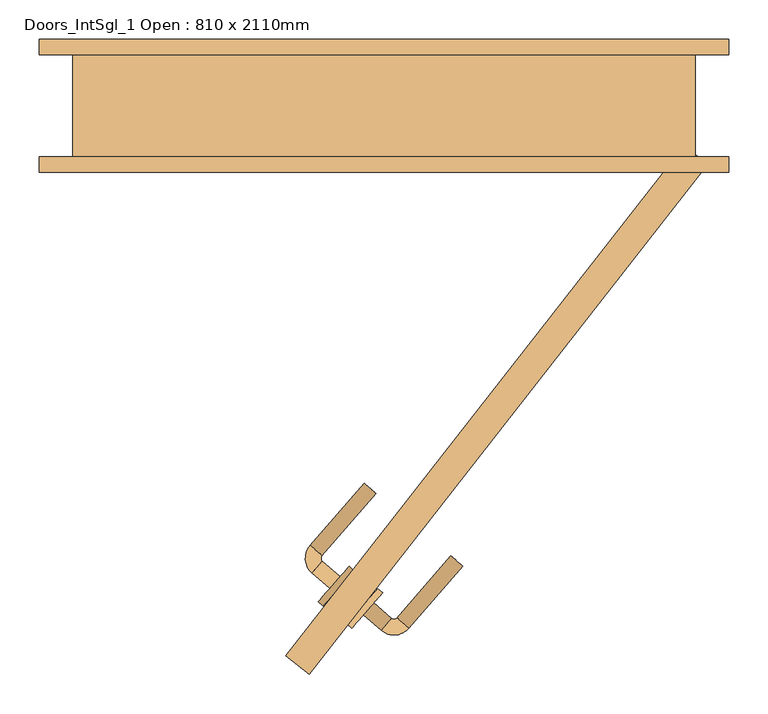
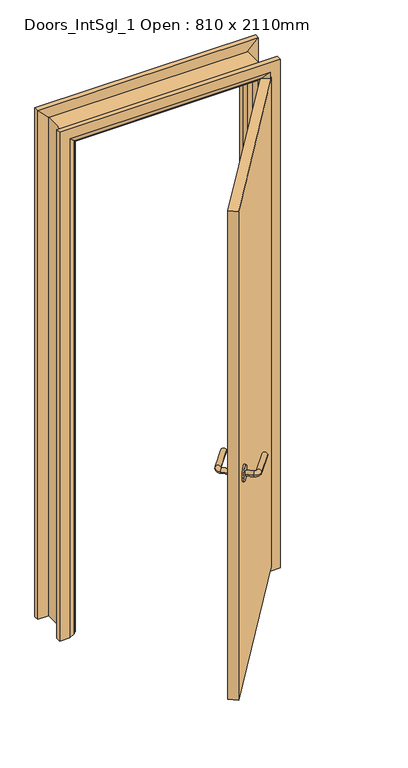
"""IFC4 building model written with IfcOpenShell, lengths in millimetres: door geometry, Doors_IntSgl_1 Open : 810 x 2110mm."""

from ifc_helpers import new_model, si_unit, point, frame, frame_2d, origin, place, context, project, spatial, polyline, circle_curve, ellipse_curve, trimmed, segment, composite_curve, outline, extrude, faceted_brep, source, transform, mapped, element, save
from ifc_brep_helpers import plane_surface, cylinder_surface, revolved_surface, advanced_brep


def doors_intsgl_1_open_810_x_2110mm_3496c895(model_context):
    return source(origin(), model_context, "Body", "SolidModel", [
        advanced_brep(
        [(-69.1197704, -615.7042456, 900.0), (-55.9985898, -600.610054, 900.0), (-91.7610578, -596.0224748, 900.0), (-78.6398772, -580.9282832, 900.0), (-79.13313, -573.8744401, 900.0), (-94.2273216, -560.7532595, 900.0), (-25.3411235, -481.5087536, 900.0), (-10.2469319, -494.6299342, 900.0)],
        [
            (0, 1, circle_curve(frame((-62.5591801, -608.1571498, 900.0), z_axis=(0.7547095802227883, -0.6560590289904886, 0.0), x_axis=(0.6560590289904885, 0.7547095802227881, 0.0)), 10.0)),
            (1, 0, circle_curve(frame((-62.5591801, -608.1571498, 900.0), z_axis=(0.7547095802227883, -0.6560590289904886, 0.0), x_axis=(0.6560590289904885, 0.7547095802227881, 0.0)), 10.0)),
            (0, 2),
            (2, 3, circle_curve(frame((-85.2004675, -588.475379, 900.0), z_axis=(0.7547095802227883, -0.6560590289904886, 0.0), x_axis=(0.6560590289904885, 0.7547095802227881, 0.0)), 10.0)),
            (3, 1),
            (3, 2, circle_curve(frame((-85.2004675, -588.475379, 900.0), z_axis=(0.7547095802227883, -0.6560590289904886, 0.0), x_axis=(0.6560590289904885, 0.7547095802227881, 0.0)), 10.0)),
            (4, 3, circle_curve(frame((-75.3595821, -577.1547353, 900.0), z_axis=(0.0, 0.0, 1.0), x_axis=(-0.6560590289904885, -0.7547095802227881, 0.0)), 5.0)),
            (2, 5, circle_curve(frame((-75.3595821, -577.1547353, 900.0), z_axis=(0.0, 0.0, -1.0), x_axis=(-0.6560590289904885, -0.7547095802227881, 0.0)), 25.0)),
            (5, 4, circle_curve(frame((-86.6802258, -567.3138498, 900.0), z_axis=(-0.656059028990488, -0.7547095802227886, 0.0), x_axis=(0.7547095802227886, -0.656059028990488, 0.0)), 10.0)),
            (4, 5, circle_curve(frame((-86.6802258, -567.3138498, 900.0), z_axis=(-0.6560590289904857, -0.7547095802227904, 0.0), x_axis=(0.7547095802227904, -0.6560590289904857, 0.0)), 10.0)),
            (6, 7, circle_curve(frame((-17.7940277, -488.0693439, 900.0), z_axis=(0.6560590289904886, 0.7547095802227883, 0.0), x_axis=(0.7547095802227881, -0.6560590289904885, 0.0)), 10.0)),
            (7, 6, circle_curve(frame((-17.7940277, -488.0693439, 900.0), z_axis=(0.6560590289904886, 0.7547095802227883, 0.0), x_axis=(0.7547095802227881, -0.6560590289904885, 0.0)), 10.0)),
            (5, 6),
            (7, 4),
        ],
        [
            plane_surface(frame((-62.5591801, -608.1571498, 900.0), z_axis=(0.7547095802227883, -0.6560590289904886, 0.0), x_axis=(0.0, 0.0, 1.0))),
            cylinder_surface(frame((-62.5591801, -608.1571498, 900.0), z_axis=(0.7547095802227881, -0.6560590289904885, 0.0), x_axis=(0.6560590289904885, 0.7547095802227881, 0.0)), 10.0),
            revolved_surface(trimmed(ellipse_curve(frame((-85.2004675, -588.475379, 900.0), z_axis=(0.7547095802227881, -0.6560590289904885, 0.0), x_axis=(0.6560590289904885, 0.7547095802227881, 0.0)), 10.0, 10.0), [point((-91.7610578, -596.0224748, 900.0))], [point((-78.6398772, -580.9282832, 900.0))], True, "CARTESIAN"), (-75.3595821, -577.1547353, 900.0), (0.0, 0.0, -1.0)),
            revolved_surface(trimmed(ellipse_curve(frame((-85.2004675, -588.475379, 900.0), z_axis=(0.7547095802227881, -0.6560590289904885, 0.0), x_axis=(0.6560590289904885, 0.7547095802227881, 0.0)), 10.0, 10.0), [point((-78.6398772, -580.9282832, 900.0))], [point((-91.7610578, -596.0224748, 900.0))], True, "CARTESIAN"), (-75.3595821, -577.1547353, 900.0), (0.0, 0.0, -1.0)),
            plane_surface(frame((-17.7940277, -488.0693439, 900.0), z_axis=(0.6560590289904886, 0.7547095802227883, 0.0), x_axis=(0.0, 0.0, 1.0))),
            cylinder_surface(frame((-86.6802258, -567.3138498, 900.0), z_axis=(-0.6560590289904885, -0.7547095802227881, 0.0), x_axis=(0.7547095802227881, -0.6560590289904885, 0.0)), 10.0),
        ],
        [
            (0, [[1, 2]]),
            (1, [[-1, 3, 4, 5]]),
            (1, [[-2, -5, 6, -3]]),
            (2, [[7, -4, 8, 9]]),
            (3, [[-8, -6, -7, 10]]),
            (4, [[11, 12]]),
            (5, [[-9, 13, -12, 14]]),
            (5, [[-10, -14, -11, -13]]),
        ],
    ),
        extrude(outline(composite_curve([segment(trimmed(circle_curve(frame_2d((0.0, -30.0)), 30.0), [point((0.0, -60.0))], [point((0.0, 0.0))], False, "CARTESIAN"), True, "CONTINUOUS"), segment(trimmed(circle_curve(frame_2d((0.0, -30.0)), 30.0), [point((0.0, 0.0))], [point((0.0, -60.0))], False, "CARTESIAN"), True, "CONTINUOUS")], self_intersect=False)), frame((-38.4798801, -592.6511086, 900.0), z_axis=(-0.7547095802227883, 0.6560590289904886, 0.0), x_axis=(0.0, 0.0, 1.0)), (0.0, 0.0, 1.0), 8.0),
        advanced_brep(
        [(-26.2647476, -649.3053178, 900.0), (-13.143567, -634.2111262, 900.0), (9.4977204, -653.8928971, 900.0), (-3.6234602, -668.9870887, 900.0), (16.5515634, -653.3996443, 900.0), (31.645755, -666.5208249, 900.0), (100.5319531, -587.276319, 900.0), (85.4377615, -574.1551384, 900.0)],
        [
            (0, 1, circle_curve(frame((-19.7041573, -641.758222, 900.0), z_axis=(-0.7547095802227883, 0.6560590289904886, 0.0), x_axis=(0.6560590289904885, 0.7547095802227881, 0.0)), 10.0)),
            (1, 0, circle_curve(frame((-19.7041573, -641.758222, 900.0), z_axis=(-0.7547095802227883, 0.6560590289904886, 0.0), x_axis=(0.6560590289904885, 0.7547095802227881, 0.0)), 10.0)),
            (1, 2),
            (2, 3, circle_curve(frame((2.9371301, -661.4399929, 900.0), z_axis=(-0.7547095802227883, 0.6560590289904886, 0.0), x_axis=(0.6560590289904885, 0.7547095802227881, 0.0)), 10.0)),
            (3, 0),
            (3, 2, circle_curve(frame((2.9371301, -661.4399929, 900.0), z_axis=(-0.7547095802227883, 0.6560590289904886, 0.0), x_axis=(0.6560590289904885, 0.7547095802227881, 0.0)), 10.0)),
            (4, 5, circle_curve(frame((24.0986592, -659.9602346, 900.0), z_axis=(-0.6560590289904913, -0.7547095802227858, 0.0), x_axis=(-0.7547095802227858, 0.6560590289904913, 0.0)), 10.0)),
            (5, 3, circle_curve(frame((12.7780155, -650.1193492, 900.0), z_axis=(0.0, 0.0, -1.0), x_axis=(-0.6560590289904885, -0.7547095802227881, 0.0)), 25.0)),
            (2, 4, circle_curve(frame((12.7780155, -650.1193492, 900.0), z_axis=(0.0, 0.0, 1.0), x_axis=(-0.6560590289904885, -0.7547095802227881, 0.0)), 5.0)),
            (5, 4, circle_curve(frame((24.0986592, -659.9602346, 900.0), z_axis=(-0.6560590289904891, -0.7547095802227877, 0.0), x_axis=(-0.7547095802227877, 0.6560590289904891, 0.0)), 10.0)),
            (6, 7, circle_curve(frame((92.9848573, -580.7157287, 900.0), z_axis=(0.6560590289904886, 0.7547095802227883, 0.0), x_axis=(-0.7547095802227881, 0.6560590289904885, 0.0)), 10.0)),
            (7, 6, circle_curve(frame((92.9848573, -580.7157287, 900.0), z_axis=(0.6560590289904886, 0.7547095802227883, 0.0), x_axis=(-0.7547095802227881, 0.6560590289904885, 0.0)), 10.0)),
            (4, 7),
            (6, 5),
        ],
        [
            plane_surface(frame((-19.7041573, -641.758222, 900.0), z_axis=(-0.7547095802227883, 0.6560590289904886, 0.0), x_axis=(0.0, 0.0, 1.0))),
            cylinder_surface(frame((-19.7041573, -641.758222, 900.0), z_axis=(-0.7547095802227881, 0.6560590289904885, 0.0), x_axis=(0.6560590289904885, 0.7547095802227881, 0.0)), 10.0),
            revolved_surface(trimmed(ellipse_curve(frame((2.9371301, -661.4399929, 900.0), z_axis=(0.7547095802227881, -0.6560590289904885, 0.0), x_axis=(0.6560590289904885, 0.7547095802227881, 0.0)), 10.0, 10.0), [point((-3.6234602, -668.9870887, 900.0))], [point((9.4977204, -653.8928971, 900.0))], True, "CARTESIAN"), (12.7780155, -650.1193492, 900.0), (0.0, 0.0, -1.0)),
            revolved_surface(trimmed(ellipse_curve(frame((2.9371301, -661.4399929, 900.0), z_axis=(0.7547095802227881, -0.6560590289904885, 0.0), x_axis=(0.6560590289904885, 0.7547095802227881, 0.0)), 10.0, 10.0), [point((9.4977204, -653.8928971, 900.0))], [point((-3.6234602, -668.9870887, 900.0))], True, "CARTESIAN"), (12.7780155, -650.1193492, 900.0), (0.0, 0.0, -1.0)),
            plane_surface(frame((92.9848573, -580.7157287, 900.0), z_axis=(0.6560590289904886, 0.7547095802227883, 0.0), x_axis=(0.0, 0.0, 1.0))),
            cylinder_surface(frame((24.0986592, -659.9602346, 900.0), z_axis=(-0.6560590289904885, -0.7547095802227881, 0.0), x_axis=(-0.7547095802227881, 0.6560590289904885, 0.0)), 10.0),
        ],
        [
            (0, [[1, 2]]),
            (1, [[3, 4, 5, -2]]),
            (1, [[-5, 6, -3, -1]]),
            (2, [[7, 8, -4, 9]]),
            (3, [[10, -9, -6, -8]]),
            (4, [[11, 12]]),
            (5, [[13, -11, 14, -7]]),
            (5, [[-14, -12, -13, -10]]),
        ],
    ),
        extrude(outline(composite_curve([segment(trimmed(circle_curve(frame_2d((0.0, 30.0)), 30.0), [point((0.0, 60.0))], [point((0.0, 0.0))], False, "CARTESIAN"), True, "CONTINUOUS"), segment(trimmed(circle_curve(frame_2d((0.0, 30.0)), 30.0), [point((0.0, 0.0))], [point((0.0, 60.0))], False, "CARTESIAN"), True, "CONTINUOUS")], self_intersect=False)), frame((-1.662534, -621.0037086, 900.0), z_axis=(-0.7547095802227883, 0.6560590289904886, 0.0), x_axis=(0.0, 0.0, -1.0)), (0.0, 0.0, 1.0), 8.0),
        extrude(outline(polyline([(383.3995748, -51.0018026), (413.3439834, -74.3969387), (-95.1923952, -725.2938212), (-125.1368039, -701.8986851), (383.3995748, -51.0018026)])), frame((0.0, 0.0, 18.0), z_axis=(0.0, 0.0, 1.0), x_axis=(1.0, 0.0, 0.0)), (0.0, 0.0, 1.0), 2060.0),
        advanced_brep(
        [(440.0, -85.0, 0.0), (400.0, -85.0, 0.0), (374.0, -71.0, 0.0), (370.0, -65.0, 0.0), (440.0, -65.0, 0.0), (440.0, -65.0, 2145.0), (440.0, -85.0, 2145.0), (370.0, -65.0, 2075.0), (-370.0, -65.0, 2075.0), (-370.0, -65.0, 0.0), (-440.0, -65.0, 0.0), (-440.0, -65.0, 2145.0), (374.0, -71.0, 2079.0), (400.0, -85.0, 2105.0), (-440.0, -85.0, 2145.0), (-440.0, -85.0, 0.0), (-400.0, -85.0, 0.0), (-400.0, -85.0, 2105.0), (-374.0, -71.0, 0.0), (-374.0, -71.0, 2079.0)],
        [
            (0, 1),
            (1, 2),
            (2, 3, circle_curve(frame((378.0, -64.0, 0.0), z_axis=(0.0, 0.0, -1.0), x_axis=(1.0, 0.0, 0.0)), 8.0622577)),
            (3, 4),
            (4, 0),
            (4, 5),
            (5, 6),
            (6, 0),
            (3, 7),
            (7, 8),
            (8, 9),
            (9, 10),
            (10, 11),
            (11, 5),
            (2, 12),
            (12, 7, ellipse_curve(frame((378.0, -64.0, 2083.0), z_axis=(0.7071067811865475, 0.0, -0.7071067811865475), x_axis=(-0.7071067811865474, 0.0, -0.7071067811865476)), 11.4017543, 8.0622577)),
            (1, 13),
            (13, 12),
            (6, 14),
            (14, 15),
            (15, 16),
            (16, 17),
            (17, 13),
            (10, 15),
            (14, 11),
            (9, 18, circle_curve(frame((-378.0, -64.0, 0.0), z_axis=(0.0, 0.0, -1.0), x_axis=(-1.0, 0.0, 0.0)), 8.0622577)),
            (18, 16),
            (19, 18),
            (8, 19, ellipse_curve(frame((-378.0, -64.0, 2083.0), z_axis=(-0.7071067811865475, 0.0, -0.7071067811865475), x_axis=(-0.7071067811865474, 0.0, 0.7071067811865476)), 11.4017543, 8.0622577)),
            (19, 17),
            (12, 19),
        ],
        [
            plane_surface(frame((370.0, -65.0, 0.0), z_axis=(0.0, 0.0, -1.0), x_axis=(0.0, 1.0, 0.0))),
            plane_surface(frame((440.0, -85.0, 0.0), z_axis=(1.0, 0.0, 0.0), x_axis=(0.0, 0.0, 1.0))),
            plane_surface(frame((440.0, -65.0, 0.0), z_axis=(0.0, 1.0, 0.0), x_axis=(0.0, 0.0, 1.0))),
            cylinder_surface(frame((378.0, -64.0, 0.0), z_axis=(0.0, 0.0, -1.0), x_axis=(1.0, 0.0, 0.0)), 8.0622577),
            plane_surface(frame((374.0, -71.0, 0.0), z_axis=(-0.4740998230350126, -0.880471099922178, 0.0), x_axis=(0.0, 0.0, 1.0))),
            plane_surface(frame((400.0, -85.0, 0.0), z_axis=(0.0, -1.0, 0.0), x_axis=(0.0, 0.0, 1.0))),
            plane_surface(frame((-440.0, -85.0, 2145.0), z_axis=(-1.0, 0.0, 0.0), x_axis=(0.0, 0.0, -1.0))),
            plane_surface(frame((-370.0, -65.0, 0.0), z_axis=(0.0, 0.0, -1.0), x_axis=(0.0, 1.0, 0.0))),
            cylinder_surface(frame((-378.0, -64.0, 2075.0), z_axis=(0.0, 0.0, 1.0), x_axis=(-1.0, 0.0, 0.0)), 8.0622577),
            plane_surface(frame((-374.0, -71.0, 2079.0), z_axis=(0.47409982303501824, -0.8804710999221749, 0.0), x_axis=(0.0, 0.0, -1.0))),
            plane_surface(frame((440.0, -85.0, 2145.0), z_axis=(0.0, 0.0, 1.0), x_axis=(-1.0, 0.0, 0.0))),
            cylinder_surface(frame((370.0, -64.0, 2083.0), z_axis=(1.0, 0.0, 0.0), x_axis=(0.0, 0.0, 1.0)), 8.0622577),
            plane_surface(frame((374.0, -71.0, 2079.0), z_axis=(0.0, -0.8804710999221764, -0.4740998230350154), x_axis=(-1.0, 0.0, 0.0))),
        ],
        [
            (0, [[1, 2, 3, 4, 5]]),
            (1, [[6, 7, 8, -5]]),
            (2, [[9, 10, 11, 12, 13, 14, -6, -4]]),
            (3, [[15, 16, -9, -3]]),
            (4, [[17, 18, -15, -2]]),
            (5, [[-8, 19, 20, 21, 22, 23, -17, -1]]),
            (6, [[-13, 24, -20, 25]]),
            (7, [[-24, -12, 26, 27, -21]]),
            (8, [[28, -26, -11, 29]]),
            (9, [[-22, -27, -28, 30]]),
            (10, [[-14, -25, -19, -7]]),
            (11, [[31, -29, -10, -16]]),
            (12, [[-23, -30, -31, -18]]),
        ],
    ),
        extrude(outline(polyline([(0.0, -346.0), (2051.0, -346.0), (2051.0, 346.0), (0.0, 346.0), (0.0, 365.0), (2070.0, 365.0), (2070.0, -365.0), (0.0, -365.0), (0.0, -346.0)])), frame((0.0, -25.0, 0.0), z_axis=(0.0, 1.0, 0.0), x_axis=(0.0, 0.0, 1.0)), (0.0, 0.0, 1.0), 32.0),
        advanced_brep(
        [(-440.0, 85.0, 0.0), (-400.0, 85.0, 0.0), (-374.0, 71.0, 0.0), (-370.0, 65.0, 0.0), (-440.0, 65.0, 0.0), (-440.0, 65.0, 2145.0), (-440.0, 85.0, 2145.0), (-370.0, 65.0, 2075.0), (-374.0, 71.0, 2079.0), (-400.0, 85.0, 2105.0), (440.0, 85.0, 0.0), (440.0, 65.0, 0.0), (370.0, 65.0, 0.0), (374.0, 71.0, 0.0), (400.0, 85.0, 0.0), (440.0, 85.0, 2145.0), (400.0, 85.0, 2105.0), (374.0, 71.0, 2079.0), (370.0, 65.0, 2075.0), (440.0, 65.0, 2145.0)],
        [
            (0, 1),
            (1, 2),
            (2, 3, circle_curve(frame((-378.0, 64.0, 0.0), z_axis=(0.0, 0.0, -1.0), x_axis=(-1.0, 0.0, 0.0)), 8.0622577)),
            (3, 4),
            (4, 0),
            (4, 5),
            (5, 6),
            (6, 0),
            (3, 7),
            (7, 5),
            (2, 8),
            (8, 7, ellipse_curve(frame((-378.0, 64.0, 2083.0), z_axis=(-0.7071067811865475, 0.0, -0.7071067811865475), x_axis=(0.7071067811865474, 0.0, -0.7071067811865476)), 11.4017543, 8.0622577)),
            (1, 9),
            (9, 8),
            (6, 9),
            (10, 11),
            (11, 12),
            (12, 13, circle_curve(frame((378.0, 64.0, 0.0), z_axis=(0.0, 0.0, -1.0), x_axis=(1.0, 0.0, 0.0)), 8.0622577)),
            (13, 14),
            (14, 10),
            (15, 10),
            (14, 16),
            (16, 15),
            (13, 17),
            (17, 16),
            (12, 18),
            (18, 17, ellipse_curve(frame((378.0, 64.0, 2083.0), z_axis=(0.7071067811865475, 0.0, -0.7071067811865475), x_axis=(0.7071067811865474, 0.0, 0.7071067811865476)), 11.4017543, 8.0622577)),
            (11, 19),
            (19, 18),
            (15, 19),
            (5, 19),
            (15, 6),
            (7, 18),
            (8, 17),
            (9, 16),
        ],
        [
            plane_surface(frame((-370.0, 137.8010989, 0.0), z_axis=(0.0, 0.0, -1.0), x_axis=(1.0, 0.0, 0.0))),
            plane_surface(frame((-440.0, 85.0, 0.0), z_axis=(-1.0, 0.0, 0.0), x_axis=(0.0, 0.0, 1.0))),
            plane_surface(frame((-440.0, 65.0, 0.0), z_axis=(0.0, -1.0, 0.0), x_axis=(0.0, 0.0, 1.0))),
            cylinder_surface(frame((-378.0, 64.0, 0.0), z_axis=(0.0, 0.0, -1.0), x_axis=(-1.0, 0.0, 0.0)), 8.0622577),
            plane_surface(frame((-374.0, 71.0, 0.0), z_axis=(0.4740998230350183, 0.8804710999221749, 0.0), x_axis=(0.0, 0.0, 1.0))),
            plane_surface(frame((-400.0, 85.0, 0.0), z_axis=(0.0, 1.0, 0.0), x_axis=(0.0, 0.0, 1.0))),
            plane_surface(frame((370.0, 137.8010989, 0.0), z_axis=(0.0, 0.0, -1.0), x_axis=(-1.0, 0.0, 0.0))),
            plane_surface(frame((400.0, 85.0, 2105.0), z_axis=(0.0, 1.0, 0.0), x_axis=(0.0, 0.0, -1.0))),
            plane_surface(frame((374.0, 71.0, 2079.0), z_axis=(-0.4740998230350183, 0.8804710999221749, 0.0), x_axis=(0.0, 0.0, -1.0))),
            cylinder_surface(frame((378.0, 64.0, 2075.0), z_axis=(0.0, 0.0, 1.0), x_axis=(1.0, 0.0, 0.0)), 8.0622577),
            plane_surface(frame((440.0, 65.0, 2145.0), z_axis=(0.0, -1.0, 0.0), x_axis=(0.0, 0.0, -1.0))),
            plane_surface(frame((440.0, 85.0, 2145.0), z_axis=(1.0, 0.0, 0.0), x_axis=(0.0, 0.0, -1.0))),
            plane_surface(frame((-440.0, 85.0, 2145.0), z_axis=(0.0, 0.0, 1.0), x_axis=(1.0, 0.0, 0.0))),
            plane_surface(frame((-440.0, 65.0, 2145.0), z_axis=(0.0, -1.0, 0.0), x_axis=(1.0, 0.0, 0.0))),
            cylinder_surface(frame((-370.0, 64.0, 2083.0), z_axis=(-1.0, 0.0, 0.0), x_axis=(0.0, 0.0, 1.0)), 8.0622577),
            plane_surface(frame((-374.0, 71.0, 2079.0), z_axis=(0.0, 0.8804710999221749, -0.4740998230350183), x_axis=(1.0, 0.0, 0.0))),
            plane_surface(frame((-400.0, 85.0, 2105.0), z_axis=(0.0, 1.0, 0.0), x_axis=(1.0, 0.0, 0.0))),
        ],
        [
            (0, [[1, 2, 3, 4, 5]]),
            (1, [[6, 7, 8, -5]]),
            (2, [[9, 10, -6, -4]]),
            (3, [[11, 12, -9, -3]]),
            (4, [[13, 14, -11, -2]]),
            (5, [[-8, 15, -13, -1]]),
            (6, [[16, 17, 18, 19, 20]]),
            (7, [[21, -20, 22, 23]]),
            (8, [[-22, -19, 24, 25]]),
            (9, [[-24, -18, 26, 27]]),
            (10, [[-26, -17, 28, 29]]),
            (11, [[-28, -16, -21, 30]]),
            (12, [[31, -30, 32, -7]]),
            (13, [[33, -29, -31, -10]]),
            (14, [[34, -27, -33, -12]]),
            (15, [[35, -25, -34, -14]]),
            (16, [[-32, -23, -35, -15]]),
        ],
    ),
        faceted_brep([(-365.0, -65.0, 0.0), (-397.0, -65.0, 0.0), (-397.0, 65.0, 0.0), (-365.0, 65.0, 0.0), (-365.0, 65.0, 2070.0), (-365.0, -65.0, 2070.0), (-397.0, 65.0, 2102.0), (-397.0, -65.0, 2102.0), (365.0, -65.0, 0.0), (365.0, 65.0, 0.0), (397.0, 65.0, 0.0), (397.0, -65.0, 0.0), (365.0, -65.0, 2070.0), (397.0, -65.0, 2102.0), (397.0, 65.0, 2102.0), (365.0, 65.0, 2070.0)], [[[0, 1, 2, 3]], [[3, 4, 5, 0]], [[2, 6, 4, 3]], [[1, 7, 6, 2]], [[0, 5, 7, 1]], [[8, 9, 10, 11]], [[12, 8, 11, 13]], [[13, 11, 10, 14]], [[14, 10, 9, 15]], [[15, 9, 8, 12]], [[4, 15, 12, 5]], [[6, 14, 15, 4]], [[7, 13, 14, 6]], [[5, 12, 13, 7]]]),
    ])


if __name__ == "__main__":
    model = new_model("IFC4")
    model_context = context("Model", 3, world=origin())
    ifc_project = project(units=[si_unit("LENGTHUNIT", "METRE", prefix="MILLI")], contexts=[model_context])
    site = spatial("IfcSite", under=ifc_project)
    building = spatial("IfcBuilding", under=site)
    placement = place(None, origin())
    doors_intsgl_1_open_810_x_2110mm_shape = doors_intsgl_1_open_810_x_2110mm_3496c895(model_context)
    element("IfcDoor", 1, ObjectType="Doors_IntSgl_1 Open : 810 x 2110mm", at=placement, inside=building, context=model_context, shape_type="MappedRepresentation", body=[
        mapped(doors_intsgl_1_open_810_x_2110mm_shape, transform((0.0, 0.0, 0.0), x_axis=(1.0, 0.0, 0.0), y_axis=(0.0, 1.0, 0.0), z_axis=(0.0, 0.0, 1.0))),
    ])
    save(model, "model.ifc")

# Revit data of these elements
# Type "Doors_IntSgl_1 Open : 810 x 2110mm"
#   Type Mark = "69"
#   Type Comments = "Internal Single"
#   Operation = "SingleSwingRight"
#   Manufacturer = "Revit"
#   Keynote = "L20"
#   Description = "Internal Single Door"
#   Analytic Construction = "Metal"
#   UnderCut = 8 mm
#   Tolerance = 2 mm
#   Thickness = 38 mm
#   Thermal Resistance (R) = 0.270117 (m²·K)/W
#   Structural Tolerance = 8 mm
#   StopDepth = 32 mm
#   Stop Thickness = 19 mm
#   Rough Width = 810 mm
#   Rough Height = 2110 mm
#   Height to Top Lock Rail = 1000 mm
#   Heat Transfer Coefficient (U) = 3.7021 W/(m²·K)
#   Handle Z Distance = 900 mm
#   Handle X Distance = 75 mm
#   Frame Thickness = 32 mm
#   Door Panel Width = 726 mm
#   Door Panel Thickness = 38 mm
#   Door Panel Offset = 0 mm
#   Height = 2110 mm
#   Width = 810 mm
#   Door Panel Height = 2060 mm
#   Architrave Setback = 5 mm
#   Vis - Ironmongery = yes
#   Material Ironmongery = Door - Handle
#   Material Frame = Door - Frame/Mullion (1)
#   Material Door = Door - Panel
#   Material Architrave = Door - Architrave
#   Visual Light Transmittance = 0
#   Solar Heat Gain Coefficient = 0
#   Function = (empty or 0)
#   Wall Closure = (empty or 0)
# Element 1 (IfcDoor, "Doors_IntSgl_1 Open : 810 x 2110mm")
#   Materials on its faces: "Door - Architrave", "Door - Handle", "Door - Frame/Mullion (1)", "Door - Panel"
# Materials
#   "Door - Handle": class "Miscellaneous", colour RGB 0 0 0, transparency 0, Keynote = "P21"
#   "Door - Frame/Mullion (1)": class "Wood", colour RGB 212 179 113, transparency 0, Keynote = "L20", Cost = 0
#   "Door - Panel": class "Wood", colour RGB 210 159 95, transparency 0, Keynote = "L20"
#   "Door - Architrave": class "Wood", colour RGB 154 90 5, transparency 0, Keynote = "P20"
